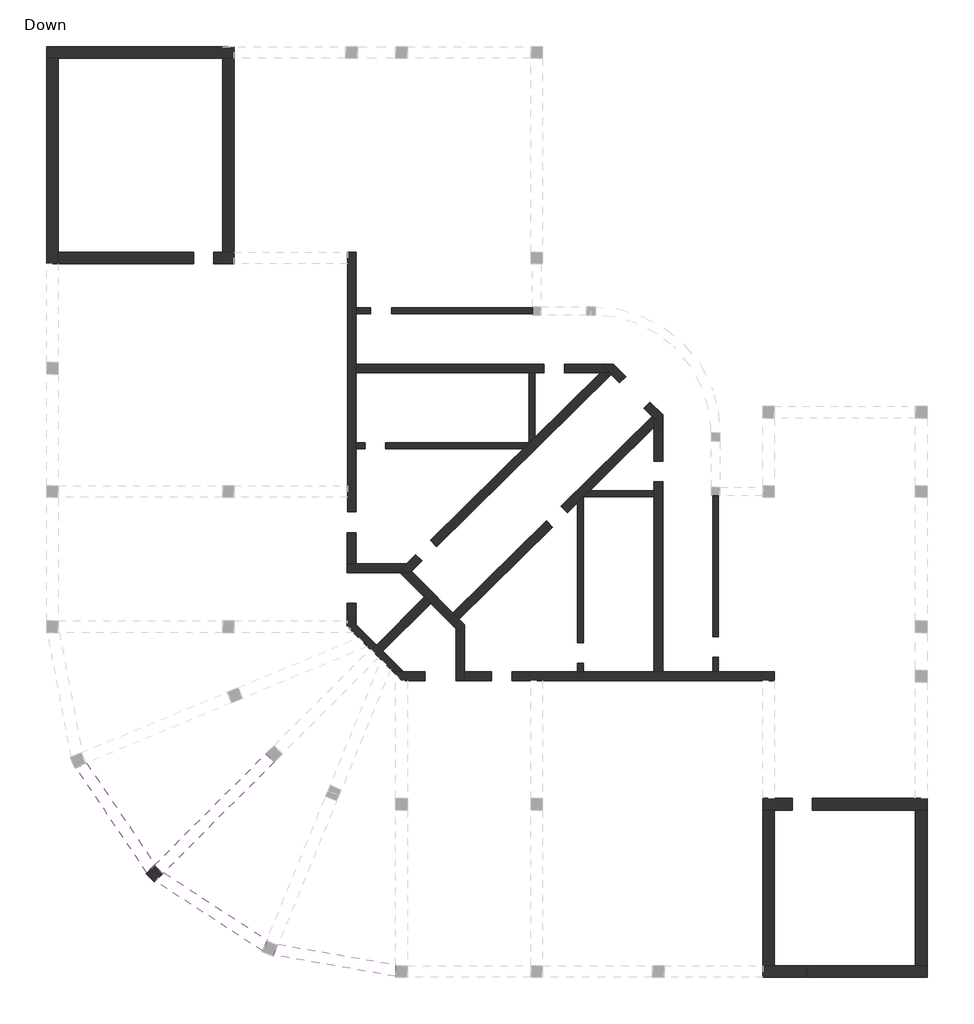
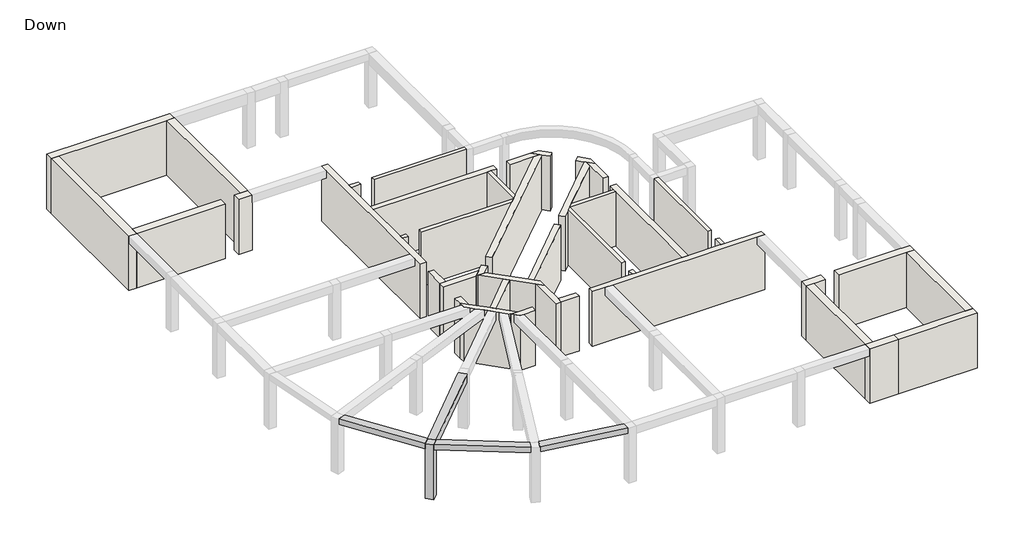
# One storey, part 1 of 2: 42 walls, 4 beams, 1 column.
# Revit data of these elements (continued)
# Element 31 (IfcWall, "30")
#   Comments = ""
#   Mark = "W28"
#   SOFiSTiK_EdgeZones = "W28"
#   SOFiSTiK_AMG_Comments = ""
#   Top Offset = 0 cm
#   Base Offset = 0 cm
#   wall height = 300 cm
#   SOFiSTiK_AMG_Scheduled = yes
#   SOFiSTiK_AMG_Adjusted = yes
#   Phase Created = New Construction
#   Base Constraint = Down
#   Top Constraint = Typical Floor
#   Materials on its faces: "Concrete"
# Element 32 (IfcWall, "30")
#   Comments = ""
#   Mark = "W29"
#   SOFiSTiK_EdgeZones = "W29"
#   SOFiSTiK_AMG_Comments = ""
#   Top Offset = 0 cm
#   Base Offset = 0 cm
#   wall height = 300 cm
#   SOFiSTiK_AMG_Scheduled = yes
#   SOFiSTiK_AMG_Adjusted = yes
#   Phase Created = New Construction
#   Base Constraint = Down
#   Top Constraint = Typical Floor
#   Materials on its faces: "Concrete"
# Element 33 (IfcWall, "30")
#   Comments = ""
#   Mark = "W30"
#   SOFiSTiK_EdgeZones = "W30"
#   SOFiSTiK_AMG_Comments = ""
#   Top Offset = 0 cm
#   Base Offset = 0 cm
#   wall height = 300 cm
#   SOFiSTiK_AMG_Scheduled = yes
#   SOFiSTiK_AMG_Adjusted = yes
#   Phase Created = New Construction
#   Base Constraint = Down
#   Top Constraint = Typical Floor
#   Materials on its faces: "Concrete"
# Element 34 (IfcWall, "30")
#   Comments = ""
#   Mark = "W31"
#   SOFiSTiK_EdgeZones = "W31"
#   SOFiSTiK_AMG_Comments = ""
#   Top Offset = 0 cm
#   Base Offset = 0 cm
#   wall height = 300 cm
#   SOFiSTiK_AMG_Scheduled = yes
#   SOFiSTiK_AMG_Adjusted = yes
#   Phase Created = New Construction
#   Base Constraint = Down
#   Top Constraint = Typical Floor
#   Materials on its faces: "Concrete"
# Element 35 (IfcWall, "30")
#   Comments = ""
#   Mark = "W32"
#   SOFiSTiK_EdgeZones = "W32"
#   SOFiSTiK_AMG_Comments = ""
#   Top Offset = 0 cm
#   Base Offset = 0 cm
#   wall height = 300 cm
#   SOFiSTiK_AMG_Scheduled = yes
#   SOFiSTiK_AMG_Adjusted = yes
#   Phase Created = New Construction
#   Base Constraint = Down
#   Top Constraint = Typical Floor
#   Materials on its faces: "Concrete"
# Element 36 (IfcWall, "30")
#   Comments = ""
#   Mark = "W33"
#   SOFiSTiK_EdgeZones = "W33"
#   SOFiSTiK_AMG_Comments = ""
#   Top Offset = 0 cm
#   Base Offset = 0 cm
#   wall height = 300 cm
#   SOFiSTiK_AMG_Scheduled = yes
#   SOFiSTiK_AMG_Adjusted = yes
#   Phase Created = New Construction
#   Base Constraint = Down
#   Top Constraint = Typical Floor
#   Materials on its faces: "Concrete"
# Element 37 (IfcWall, "40")
#   Comments = ""
#   Mark = "W2"
#   SOFiSTiK_EdgeZones = "W2"
#   SOFiSTiK_AMG_Comments = ""
#   Top Offset = 0 cm
#   Base Offset = 0 cm
#   wall height = 300 cm
#   SOFiSTiK_AMG_Scheduled = yes
#   SOFiSTiK_AMG_Adjusted = yes
#   Phase Created = New Construction
#   Base Constraint = Down
#   Top Constraint = Typical Floor
#   Materials on its faces: "Concrete"
# Element 38 (IfcWall, "40")
#   Comments = ""
#   Mark = "W3"
#   SOFiSTiK_EdgeZones = "W3"
#   SOFiSTiK_AMG_Comments = ""
#   Top Offset = 0 cm
#   Base Offset = 0 cm
#   wall height = 300 cm
#   SOFiSTiK_AMG_Scheduled = yes
#   SOFiSTiK_AMG_Adjusted = yes
#   Phase Created = New Construction
#   Base Constraint = Down
#   Top Constraint = Typical Floor
#   Materials on its faces: "Concrete"
# Element 39 (IfcWall, "40")
#   Comments = ""
#   Mark = "W4"
#   SOFiSTiK_EdgeZones = "W4"
#   SOFiSTiK_AMG_Comments = ""
#   Top Offset = 0 cm
#   Base Offset = 0 cm
#   wall height = 300 cm
#   SOFiSTiK_AMG_Scheduled = yes
#   SOFiSTiK_AMG_Adjusted = yes
#   Phase Created = New Construction
#   Base Constraint = Down
#   Top Constraint = Typical Floor
#   Materials on its faces: "Concrete"
# Element 40 (IfcWall, "40")
#   Comments = ""
#   Mark = "W5"
#   SOFiSTiK_EdgeZones = "W5"
#   SOFiSTiK_AMG_Comments = ""
#   Top Offset = 0 cm
#   Base Offset = 0 cm
#   wall height = 300 cm
#   SOFiSTiK_AMG_Scheduled = yes
#   SOFiSTiK_AMG_Adjusted = yes
#   Phase Created = New Construction
#   Base Constraint = Down
#   Top Constraint = Typical Floor
#   Materials on its faces: "Concrete"
# Element 41 (IfcWall, "40")
#   Comments = ""
#   Mark = "W6"
#   SOFiSTiK_EdgeZones = "W6"
#   SOFiSTiK_AMG_Comments = ""
#   Top Offset = 0 cm
#   Base Offset = 0 cm
#   wall height = 300 cm
#   SOFiSTiK_AMG_Scheduled = yes
#   SOFiSTiK_AMG_Adjusted = yes
#   Phase Created = New Construction
#   Base Constraint = Down
#   Top Constraint = Typical Floor
#   Materials on its faces: "Concrete"
# Element 42 (IfcWall, "40")
#   Comments = ""
#   Mark = "W7"
#   SOFiSTiK_EdgeZones = "W7"
#   SOFiSTiK_AMG_Comments = ""
#   Top Offset = 0 cm
#   Base Offset = 0 cm
#   wall height = 300 cm
#   SOFiSTiK_AMG_Scheduled = yes
#   SOFiSTiK_AMG_Adjusted = yes
#   Phase Created = New Construction
#   Base Constraint = Down
#   Top Constraint = Typical Floor
#   Materials on its faces: "Concrete"
# Element 43 (IfcWall, "40")
#   Comments = ""
#   Mark = "W8"
#   SOFiSTiK_EdgeZones = "W8"
#   SOFiSTiK_AMG_Comments = ""
#   Top Offset = 0 cm
#   Base Offset = 0 cm
#   wall height = 300 cm
#   SOFiSTiK_AMG_Scheduled = yes
#   SOFiSTiK_AMG_Adjusted = yes
#   Phase Created = New Construction
#   Base Constraint = Down
#   Top Constraint = Typical Floor
#   Materials on its faces: "Concrete"
# Element 44 (IfcWall, "40")
#   Comments = ""
#   Mark = "W9"
#   SOFiSTiK_EdgeZones = "W9"
#   SOFiSTiK_AMG_Comments = ""
#   Top Offset = 0 cm
#   Base Offset = 0 cm
#   wall height = 300 cm
#   SOFiSTiK_AMG_Scheduled = yes
#   SOFiSTiK_AMG_Adjusted = yes
#   Phase Created = New Construction
#   Base Constraint = Down
#   Top Constraint = Typical Floor
#   Materials on its faces: "Concrete"
# Element 45 (IfcWall, "40")
#   Comments = ""
#   Mark = "W10"
#   SOFiSTiK_EdgeZones = "W10"
#   SOFiSTiK_AMG_Comments = ""
#   Top Offset = 0 cm
#   Base Offset = 0 cm
#   wall height = 300 cm
#   SOFiSTiK_AMG_Scheduled = yes
#   SOFiSTiK_AMG_Adjusted = yes
#   Phase Created = New Construction
#   Base Constraint = Down
#   Top Constraint = Typical Floor
#   Materials on its faces: "Concrete"
# Element 46 (IfcWall, "40")
#   Comments = ""
#   Mark = "W11"
#   SOFiSTiK_EdgeZones = "W11"
#   SOFiSTiK_AMG_Comments = ""
#   Top Offset = 0 cm
#   Base Offset = 0 cm
#   wall height = 300 cm
#   SOFiSTiK_AMG_Scheduled = yes
#   SOFiSTiK_AMG_Adjusted = yes
#   Phase Created = New Construction
#   Base Constraint = Down
#   Top Constraint = Typical Floor
#   Materials on its faces: "Concrete"
# Element 47 (IfcWall, "40")
#   Comments = ""
#   Mark = "W12"
#   SOFiSTiK_EdgeZones = "W12"
#   SOFiSTiK_AMG_Comments = ""
#   Top Offset = 0 cm
#   Base Offset = 0 cm
#   wall height = 300 cm
#   SOFiSTiK_AMG_Scheduled = yes
#   SOFiSTiK_AMG_Adjusted = yes
#   Phase Created = New Construction
#   Base Constraint = Down
#   Top Constraint = Typical Floor
#   Materials on its faces: "Concrete"
# Materials
#   "Concrete": class "Concrete", colour RGB 192 192 192, transparency 0, Keynote = "01000", Description = "Cast-in-place concrete", Cost = 0
